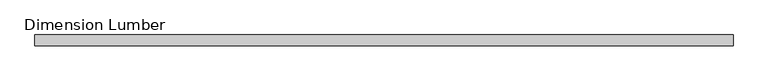
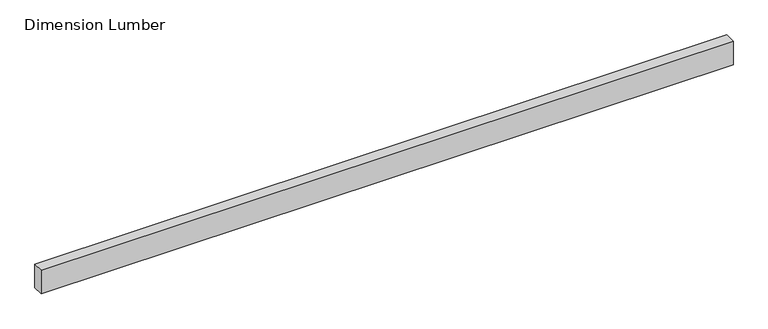
"""IFC4 building model written with IfcOpenShell, lengths in millimetres: beam geometry, Dimension Lumber : Roof Lumbers."""

from ifc_helpers import new_model, si_unit, frame, origin, place, context, project, spatial, polyline, outline, extrude, source, transform, mapped, element, save


def dimension_lumber_a2ec78f1(model_context):
    return source(origin(), model_context, "Body", "SweptSolid", [
        extrude(outline(polyline([(1250.4988621, -19.05), (-1215.9128821, -19.05), (-1215.9128821, 19.05), (1250.4988621, 19.05), (1250.4988621, -19.05)])), frame((0.0, 0.0, -44.45), z_axis=(0.0, 0.0, 1.0), x_axis=(1.0, 0.0, 0.0)), (0.0, 0.0, 1.0), 88.9),
    ])


if __name__ == "__main__":
    model = new_model("IFC4")
    model_context = context("Model", 3, world=origin())
    ifc_project = project(units=[si_unit("LENGTHUNIT", "METRE", prefix="MILLI")], contexts=[model_context])
    site = spatial("IfcSite", under=ifc_project)
    building = spatial("IfcBuilding", under=site)
    placement = place(None, origin())
    dimension_lumber_shape = dimension_lumber_a2ec78f1(model_context)
    element("IfcBeam", 1, ObjectType="Dimension Lumber : Roof Lumbers", at=placement, inside=building, context=model_context, shape_type="MappedRepresentation", body=[
        mapped(dimension_lumber_shape, transform((0.0, 0.0, 0.0), x_axis=(1.0, 0.0, 0.0), y_axis=(0.0, 1.0, 0.0), z_axis=(0.0, 0.0, 1.0))),
    ])
    save(model, "model.ifc")

# Revit data of these elements
# Type "Dimension Lumber : Roof Lumbers"
#   Assembly Code = "B10"
#   A = 0.0364583 SF
#   Length [instance default] = 5' - 0"
#   b = 0' - 1 1/2"
#   d = 0' - 3 1/2"
#   Structural Material [instance default] = Softwood, Lumber
# Element 1 (IfcBeam, "Dimension Lumber : Roof Lumbers")
#   Materials on its faces: "Softwood, Lumber"
# Materials
#   "Softwood, Lumber": class "Wood", colour RGB 223 192 134, transparency 0, Description = "Pinus Echinata", Cost = 0
